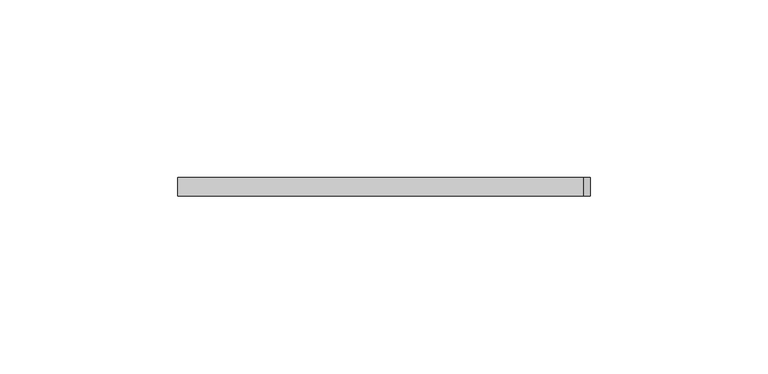
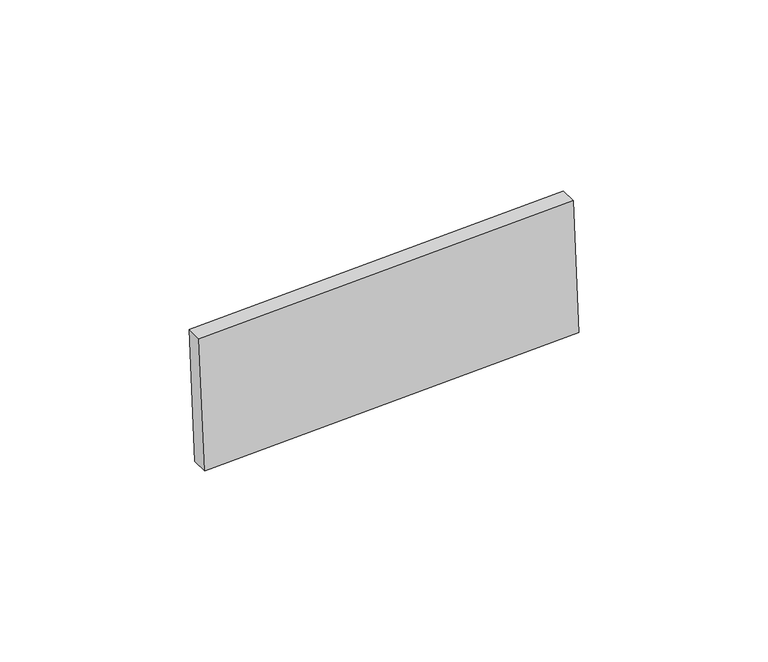
"""IFC4 building model written with IfcOpenShell, lengths in millimetres: proxy geometry, Inner panel:Inner panel:1:Inner panel:1 : Inner panel:Inner panel:300324:2:Inner panel:1:Inner panel:1 : Inner panel:Inner panel:300324:2 : Inner panel:Inner panel:1:Inner panel:1 : Inner panel:Inner panel:300324:300043:165 : Inner panel:Inner panel:1:Inner panel:1 : Inner panel:Inner panel:300324:2:Inner panel:1:Inner panel:1 : Inner panel:Inner panel:300324:2 : Inner panel:Inner panel:1:Inner panel:1 : Inner panel:Inner panel:300324:300043:308120."""

import ifcopenshell
import ifcopenshell.guid

model = None  # the IFC model being written
_history = None  # IfcOwnerHistory: only IFC2X3 demands one
_inside = {}  # id of a spatial element -> (the spatial element, [elements in it])
_under = {}  # id of a project, library or spatial element -> (it, [spatial elements below it])
_declared = {}  # id of a project -> (the project, [libraries it declares])
_typed = {}  # id of a type object -> (the type object, [elements of that type])
_made_of = {}  # id of a material, layer set ... -> (it, [elements and type objects made of it])


def new_model(schema):
    """Start an empty IFC model of exactly this schema.

    Asked for "IFC4X3", IfcOpenShell would pick the latest addendum, in which some entities
    have other attributes; the version numbers below select the first issue.
    IFC2X3 requires an IfcOwnerHistory on every rooted entity: one is made here for all.
    """
    global model, _history
    if schema == "IFC4X3":
        model = ifcopenshell.file(schema_version=(4, 3, 0, 0))
    else:
        model = ifcopenshell.file(schema=schema)
    _inside.clear()
    _under.clear()
    _declared.clear()
    _typed.clear()
    _made_of.clear()
    _history = None
    if model.schema == "IFC2X3":
        org = make("IfcOrganization", Name="unknown")
        user = make(
            "IfcPersonAndOrganization",
            ThePerson=make("IfcPerson", FamilyName="unknown"),
            TheOrganization=org,
        )
        app = make(
            "IfcApplication",
            ApplicationDeveloper=org,
            Version="unknown",
            ApplicationFullName="unknown",
            ApplicationIdentifier="unknown",
        )
        _history = make(
            "IfcOwnerHistory",
            OwningUser=user,
            OwningApplication=app,
            ChangeAction="ADDED",
            CreationDate=0,
        )
    return model


def make(cls, **values):
    """One entity of the class cls with the attributes given. An attribute that is None is left unset."""
    return model.create_entity(
        cls, **{name: value for name, value in values.items() if value is not None}
    )


def rooted(cls, **values):
    """An entity with a GlobalId (a new one), such as an element, a storey or a relation."""
    return make(cls, GlobalId=ifcopenshell.guid.new(), OwnerHistory=_history, **values)


def si_unit(unit_type, name, prefix=None):
    """IfcSIUnit, for example si_unit("LENGTHUNIT", "METRE", prefix="MILLI")."""
    return make("IfcSIUnit", UnitType=unit_type, Prefix=prefix, Name=name)


def assignment(units):
    """IfcUnitAssignment: the units of a project."""
    return None if units is None else make("IfcUnitAssignment", Units=units)


def point(xyz):
    """IfcCartesianPoint."""
    return None if xyz is None else make("IfcCartesianPoint", Coordinates=xyz)


def direction(xyz):
    """IfcDirection."""
    return None if xyz is None else make("IfcDirection", DirectionRatios=xyz)


def frame(location, z_axis=None, x_axis=None):
    """IfcAxis2Placement3D, a coordinate frame: its origin and axes. An axis left out is left unset."""
    return make(
        "IfcAxis2Placement3D",
        Location=point(location),
        Axis=direction(z_axis),
        RefDirection=direction(x_axis),
    )


def origin():
    """The frame at (0, 0, 0) with its axes left unset."""
    return frame((0.0, 0.0, 0.0))


def place(relative_to, where):
    """IfcLocalPlacement: puts the frame where relative to a parent placement (None: the world)."""
    return make(
        "IfcLocalPlacement", PlacementRelTo=relative_to, RelativePlacement=where
    )


def context(
    kind, dimensions, precision=None, world=None, true_north=None, identifier=None
):
    """IfcGeometricRepresentationContext, for example the 3D "Model" context."""
    return make(
        "IfcGeometricRepresentationContext",
        ContextIdentifier=identifier,
        ContextType=kind,
        CoordinateSpaceDimension=dimensions,
        Precision=precision,
        WorldCoordinateSystem=world,
        TrueNorth=true_north,
    )


def project(units=None, contexts=None):
    """IfcProject with its units and contexts."""
    return rooted(
        "IfcProject",
        Name="project",
        RepresentationContexts=contexts,
        UnitsInContext=assignment(units),
    )


def spatial(cls, under=None, at=None, **own):
    """A site, building, storey or space (cls), placed at a placement, below another one or the project."""
    s = rooted(cls, ObjectPlacement=at, **own)
    if under is not None:
        _under.setdefault(under.id(), (under, []))[1].append(s)
    return s


def polyline(points):
    """IfcPolyline through the points."""
    return make("IfcPolyline", Points=[point(p) for p in points])


def outline(outer, holes=None, kind="AREA"):
    """IfcArbitraryClosedProfileDef: a profile drawn as a closed curve; with holes, ...WithVoids."""
    if holes is None:
        return make("IfcArbitraryClosedProfileDef", ProfileType=kind, OuterCurve=outer)
    return make(
        "IfcArbitraryProfileDefWithVoids",
        ProfileType=kind,
        OuterCurve=outer,
        InnerCurves=holes,
    )


def extrude(swept, where, along, depth):
    """IfcExtrudedAreaSolid: the profile swept, set in the frame where, extruded along a direction by depth."""
    return make(
        "IfcExtrudedAreaSolid",
        SweptArea=swept,
        Position=where,
        ExtrudedDirection=direction(along),
        Depth=depth,
    )


def shape(context_of_items, identifier, shape_type, items):
    """IfcShapeRepresentation: the items that make up one representation, for example the "Body"."""
    return make(
        "IfcShapeRepresentation",
        ContextOfItems=context_of_items,
        RepresentationIdentifier=identifier,
        RepresentationType=shape_type,
        Items=items,
    )


def source(mapping_origin, context_of_items, identifier, shape_type, items):
    """IfcRepresentationMap: a shape defined once, which mapped items show again and again."""
    return make(
        "IfcRepresentationMap",
        MappingOrigin=mapping_origin,
        MappedRepresentation=shape(context_of_items, identifier, shape_type, items),
    )


def transform(
    local_origin,
    x_axis=None,
    y_axis=None,
    z_axis=None,
    scale=None,
    scale2=None,
    scale3=None,
    uniform=True,
):
    """IfcCartesianTransformationOperator3D, or its non-uniform kind. x_axis, y_axis, z_axis: its Axis1, 2, 3."""
    if uniform:
        return make(
            "IfcCartesianTransformationOperator3D",
            Axis1=direction(x_axis),
            Axis2=direction(y_axis),
            LocalOrigin=point(local_origin),
            Scale=scale,
            Axis3=direction(z_axis),
        )
    return make(
        "IfcCartesianTransformationOperator3DnonUniform",
        Axis1=direction(x_axis),
        Axis2=direction(y_axis),
        LocalOrigin=point(local_origin),
        Scale=scale,
        Axis3=direction(z_axis),
        Scale2=scale2,
        Scale3=scale3,
    )


def mapped(mapping_source, mapping_target):
    """IfcMappedItem: shows the shape of a source again, moved by a transform."""
    return make(
        "IfcMappedItem", MappingSource=mapping_source, MappingTarget=mapping_target
    )


def made_of(thing, what):
    """Note that an element or type object is made of a material, layer set ...; save() writes the relation."""
    if what is not None:
        _made_of.setdefault(what.id(), (what, []))[1].append(thing)
    return thing


def element(
    cls,
    number,
    at=None,
    inside=None,
    cuts=None,
    type_object=None,
    material=None,
    context=None,
    identifier="Body",
    shape_type=None,
    held_by="IfcProductDefinitionShape",
    body=None,
    shapes=None,
    **own,
):
    """One element of the class cls, such as IfcWall. Its Tag is "e" and its number.

    at: its placement. inside: the storey or other place that contains it. cuts: it is an
    opening in that element (IfcRelVoidsElement). A single representation is given by context,
    identifier, shape_type and body (its items); several are given by shapes. held_by: the class
    of the entity that holds the representations. save() writes the other relations.
    """
    e = rooted(cls, Tag="e%d" % number, ObjectPlacement=at, **own)
    if body is not None:
        shapes = [shape(context, identifier, shape_type, body)]
    if shapes is not None:
        e.Representation = make(held_by, Representations=shapes)
    if inside is not None:
        _inside.setdefault(inside.id(), (inside, []))[1].append(e)
    if cuts is not None:
        rooted(
            "IfcRelVoidsElement", RelatingBuildingElement=cuts, RelatedOpeningElement=e
        )
    if type_object is not None:
        _typed.setdefault(type_object.id(), (type_object, []))[1].append(e)
    return made_of(e, material)


def aggregate(whole, parts):
    """IfcRelAggregates: a whole, such as a stair, and the parts it consists of."""
    return rooted("IfcRelAggregates", RelatingObject=whole, RelatedObjects=parts)


def save(model, path):
    """Write the relations noted so far, then the file.

    IfcRelAggregates (storeys below a building ...), IfcRelContainedInSpatialStructure (elements
    in a storey), IfcRelDefinesByType, IfcRelAssociatesMaterial and IfcRelDeclares: one each for
    every whole, place, type object, material and project.
    """
    for whole, parts in _under.values():
        aggregate(whole, parts)
    for where, things in _inside.values():
        rooted(
            "IfcRelContainedInSpatialStructure",
            RelatedElements=things,
            RelatingStructure=where,
        )
    for kind, things in _typed.values():
        rooted("IfcRelDefinesByType", RelatedObjects=things, RelatingType=kind)
    for what, things in _made_of.values():
        rooted("IfcRelAssociatesMaterial", RelatedObjects=things, RelatingMaterial=what)
    for by, libraries in _declared.values():
        rooted("IfcRelDeclares", RelatingContext=by, RelatedDefinitions=libraries)
    model.write(path)


def generic_models_8187699f(model_context):
    return source(origin(), model_context, "Body", "SweptSolid", [
        extrude(outline(polyline([(0.0, -114.3), (0.0, 0.0), (5.213809, 0.0), (5.213809, -114.3), (0.0, -114.3)])), frame((560425.2415304, -564181.307991, 3954.8593665), z_axis=(-0.04163054471216399, 0.0, 0.9991330730923527), x_axis=(0.0, -1.0, 0.0)), (0.0, 0.0, 1.0), 43.2233908),
    ])


if __name__ == "__main__":
    model = new_model("IFC4")
    model_context = context("Model", 3, world=origin())
    ifc_project = project(units=[si_unit("LENGTHUNIT", "METRE", prefix="MILLI")], contexts=[model_context])
    site = spatial("IfcSite", under=ifc_project)
    building = spatial("IfcBuilding", under=site)
    placement = place(None, origin())
    generic_models_shape = generic_models_8187699f(model_context)
    element("IfcBuildingElementProxy", 1, Name="Inner panel:Inner panel:1:Inner panel:1 : Inner panel:Inner panel:300324:2:Inner panel:1:Inner panel:1 : Inner panel:Inner panel:300324:2 : Inner panel:Inner panel:1:Inner panel:1 : Inner panel:Inner panel:300324:300043:165 : Inner panel:Inner panel:1:Inner panel:1 : Inner panel:Inner panel:300324:2:Inner panel:1:Inner panel:1 : Inner panel:Inner panel:300324:2 : Inner panel:Inner panel:1:Inner panel:1 : Inner panel:Inner panel:300324:300043:308120", ObjectType="Inner panel:Inner panel:1:Inner panel:1 : Inner panel:Inner panel:300324:2:Inner panel:1:Inner panel:1 : Inner panel:Inner panel:300324:2 : Inner panel:Inner panel:1:Inner panel:1 : Inner panel:Inner panel:300324:300043:165 : Inner panel:Inner panel:1:Inner panel:1 : Inner panel:Inner panel:300324:2:Inner panel:1:Inner panel:1 : Inner panel:Inner panel:300324:2 : Inner panel:Inner panel:1:Inner panel:1 : Inner panel:Inner panel:300324:300043:308120", at=placement, inside=building, context=model_context, shape_type="MappedRepresentation", body=[
        mapped(generic_models_shape, transform((0.0, 0.0, 0.0), x_axis=(1.0, 0.0, 0.0), y_axis=(0.0, 1.0, 0.0), z_axis=(0.0, 0.0, 1.0))),
    ])
    save(model, "model.ifc")

# Revit data of these elements
# Type "Inner panel:Inner panel:1:Inner panel:1 : Inner panel:Inner panel:300324:2:Inner panel:1:Inner panel:1 : Inner panel:Inner panel:300324:2 : Inner panel:Inner panel:1:Inner panel:1 : Inner panel:Inner panel:300324:300043:165 : Inner panel:Inner panel:1:Inner panel:1 : Inner panel:Inner panel:300324:2:Inner panel:1:Inner panel:1 : Inner panel:Inner panel:300324:2 : Inner panel:Inner panel:1:Inner panel:1 : Inner panel:Inner panel:300324:300043:308120"
#   NameOverride = "Inner panel:Inner panel:1:Inner panel:1 : Inner panel:Inner panel:300324:2:Inner panel:1:Inner panel:1 : Inner panel:Inner panel:300324:2 : Inner panel:Inner panel:1:Inner panel:1 : Inner panel:Inner panel:300324:300043:308120"
#   ObjectTypeOverride = "Inner panel:1:Inner panel:1 : Inner panel:Inner panel:300324:2 : Inner panel:Inner panel:1:Inner panel:1 : Inner panel:Inner panel:300324:300043"
#   Reference = "Inner panel"
#   Tag = "308120"
# Element 1 (IfcBuildingElementProxy, "Inner panel:Inner panel:1:Inner panel:1 : Inner panel:Inner panel:300324:2:Inner panel:1:Inner panel:1 : Inner panel:Inner panel:300324:2 : Inner panel:Inner panel:1:Inner panel:1 : Inner panel:Inner panel:300324:300043:165 : Inner panel:Inner panel:1:Inner panel:1 : Inner panel:Inner panel:300324:2:Inner panel:1:Inner panel:1 : Inner panel:Inner panel:300324:2 : Inner panel:Inner panel:1:Inner panel:1 : Inner panel:Inner panel:300324:300043:308120")
#   Materials on its faces: "SLIDING CLIP"
# Materials
#   "SLIDING CLIP": class "Generic", colour RGB 120 120 120, transparency 0, Cost = 0
